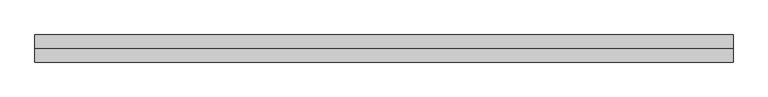
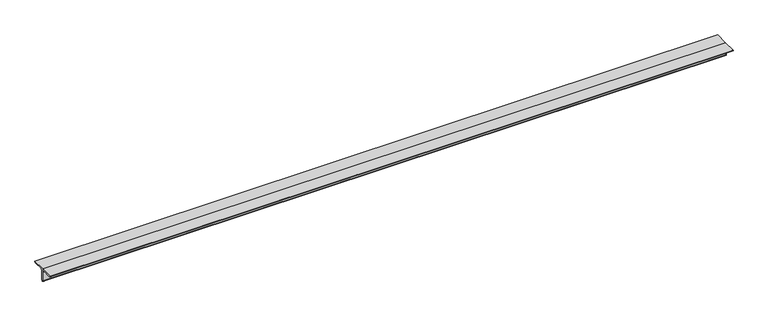
"""IFC4 building model written with IfcOpenShell, lengths in millimetres: member geometry, Steel Framing_2Ls_KS : H_SB_AR_S02_2Ls-100x100x10_VBR1."""

from ifc_helpers import new_model, si_unit, point, frame, frame_2d, origin, place, context, project, spatial, polyline, circle_curve, trimmed, segment, composite_curve, outline, extrude, source, transform, mapped, element, save


def member_612c089f(model_context):
    return source(origin(), model_context, "Body", "SweptSolid", [
        extrude(outline(composite_curve([segment(polyline([(0.0, 28.2), (100.0, 28.2)]), True, "CONTINUOUS"), segment(trimmed(circle_curve(frame_2d((90.0, 28.2)), 10.0), [point((100.0, 28.2))], [point((90.0, 18.2))], False, "CARTESIAN"), True, "CONTINUOUS"), segment(polyline([(90.0, 18.2), (20.0, 18.2)]), True, "CONTINUOUS"), segment(trimmed(circle_curve(frame_2d((20.0, 8.2)), 10.0), [point((20.0, 18.2))], [point((10.0, 8.2))], True, "CARTESIAN"), True, "CONTINUOUS"), segment(polyline([(10.0, 8.2), (10.0, -61.8)]), True, "CONTINUOUS"), segment(trimmed(circle_curve(frame_2d((0.0, -61.8)), 10.0), [point((10.0, -61.8))], [point((0.0, -71.8))], False, "CARTESIAN"), True, "CONTINUOUS"), segment(polyline([(0.0, -71.8), (0.0, 28.2)]), True, "CONTINUOUS")], self_intersect=False)), frame((-2600.492603, 0.0, 0.0), z_axis=(1.0, 0.0, 0.0), x_axis=(0.0, 1.0, 0.0)), (0.0, 0.0, 1.0), 5152.5727888),
        extrude(outline(composite_curve([segment(polyline([(0.0, 28.2), (0.0, -71.8)]), True, "CONTINUOUS"), segment(trimmed(circle_curve(frame_2d((0.0, -61.8)), 10.0), [point((0.0, -71.8))], [point((-10.0, -61.8))], False, "CARTESIAN"), True, "CONTINUOUS"), segment(polyline([(-10.0, -61.8), (-10.0, 8.2)]), True, "CONTINUOUS"), segment(trimmed(circle_curve(frame_2d((-20.0, 8.2)), 10.0), [point((-10.0, 8.2))], [point((-20.0, 18.2))], True, "CARTESIAN"), True, "CONTINUOUS"), segment(polyline([(-20.0, 18.2), (-90.0, 18.2)]), True, "CONTINUOUS"), segment(trimmed(circle_curve(frame_2d((-90.0, 28.2)), 10.0), [point((-90.0, 18.2))], [point((-100.0, 28.2))], False, "CARTESIAN"), True, "CONTINUOUS"), segment(polyline([(-100.0, 28.2), (0.0, 28.2)]), True, "CONTINUOUS")], self_intersect=False)), frame((-2600.492603, 0.0, 0.0), z_axis=(1.0, 0.0, 0.0), x_axis=(0.0, 1.0, 0.0)), (0.0, 0.0, 1.0), 5152.5727888),
    ])


if __name__ == "__main__":
    model = new_model("IFC4")
    model_context = context("Model", 3, world=origin())
    ifc_project = project(units=[si_unit("LENGTHUNIT", "METRE", prefix="MILLI")], contexts=[model_context])
    site = spatial("IfcSite", under=ifc_project)
    building = spatial("IfcBuilding", under=site)
    placement = place(None, origin())
    member_shape = member_612c089f(model_context)
    element("IfcMember", 1, ObjectType="Steel Framing_2Ls_KS : H_SB_AR_S02_2Ls-100x100x10_VBR1", at=placement, inside=building, context=model_context, shape_type="MappedRepresentation", body=[
        mapped(member_shape, transform((0.0, 0.0, 0.0), x_axis=(1.0, 0.0, 0.0), y_axis=(0.0, 1.0, 0.0), z_axis=(0.0, 0.0, 1.0))),
    ])
    save(model, "model.ifc")

# Revit data of these elements
# Type "Steel Framing_2Ls_KS : H_SB_AR_S02_2Ls-100x100x10_VBR1"
#   Type Comments = "MAIN"
#   Type Mark = "VBR1"
#   H_SectionID = "2Ls-100x100x10"
#   Assembly Code = "B10"
#   Legs = "LLBB"
#   H_Ratio for Additional Steel Plate = 0.2
#   W = 0
#   Perimeter = 0.80 m²/m
#   Nominal Weight = 29.80 kgf/m
#   Length [instance default] = 1524 mm
#   Space = 0 mm
#   b = 100 mm
#   d = 100 mm
#   t = 10 mm
#   y = 28.2 mm
#   A = 0.0038 m²
#   Structural Material [instance default] = Steel, 45-345
# Element 1 (IfcMember, "Steel Framing_2Ls_KS : H_SB_AR_S02_2Ls-100x100x10_VBR1")
#   Materials on its faces: "Steel, 45-345"
# Materials
#   "Steel, 45-345": class "Metal", colour RGB 189 187 185, transparency 0, Description = "Steel 345 MPa", Cost = 0
